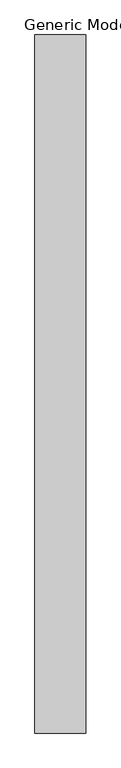
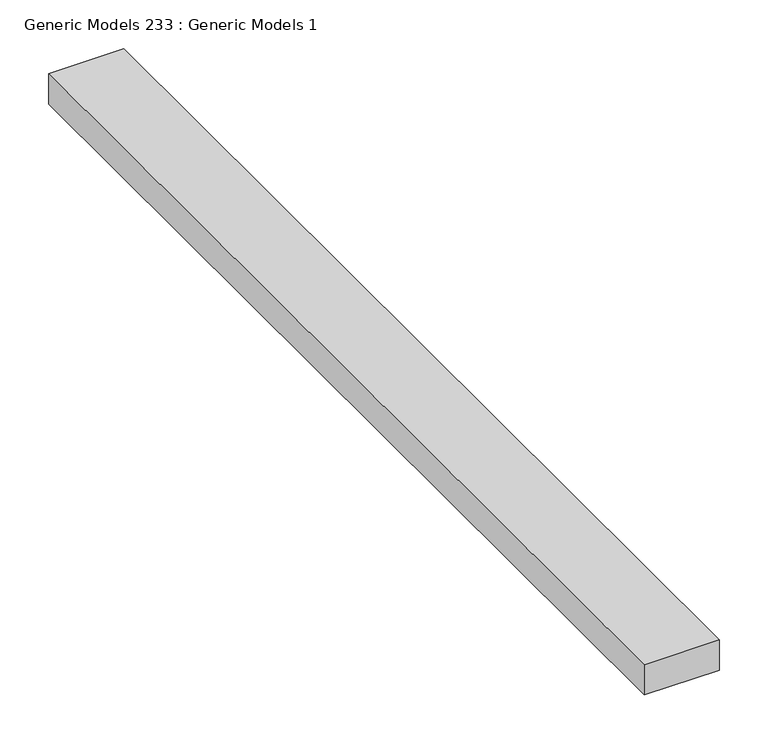
"""IFC4 building model written with IfcOpenShell, lengths in millimetres: proxy geometry, Generic Models 233 : Generic Models 1."""

from ifc_helpers import new_model, si_unit, frame, origin, place, context, project, spatial, polyline, outline, extrude, source, transform, mapped, element, save


def generic_models_233_generic_models_1_ae5bae41(model_context):
    return source(origin(), model_context, "Body", "SweptSolid", [
        extrude(outline(polyline([(48564.8, 0.0), (48475.9, 0.0), (48475.9, 1219.2), (48564.8, 1219.2), (48564.8, 0.0)])), frame((0.0, 0.0, 5467.35), z_axis=(0.0, 0.0, 1.0), x_axis=(1.0, 0.0, 0.0)), (0.0, 0.0, 1.0), 38.1),
    ])


if __name__ == "__main__":
    model = new_model("IFC4")
    model_context = context("Model", 3, world=origin())
    ifc_project = project(units=[si_unit("LENGTHUNIT", "METRE", prefix="MILLI")], contexts=[model_context])
    site = spatial("IfcSite", under=ifc_project)
    building = spatial("IfcBuilding", under=site)
    placement = place(None, origin())
    generic_models_233_generic_models_1_shape = generic_models_233_generic_models_1_ae5bae41(model_context)
    element("IfcBuildingElementProxy", 1, Name="Generic Models 233 : Generic Models 1", ObjectType="Generic Models 233 : Generic Models 1", at=placement, inside=building, context=model_context, shape_type="MappedRepresentation", body=[
        mapped(generic_models_233_generic_models_1_shape, transform((0.0, 0.0, 0.0), x_axis=(1.0, 0.0, 0.0), y_axis=(0.0, 1.0, 0.0), z_axis=(0.0, 0.0, 1.0))),
    ])
    save(model, "model.ifc")

# Revit data of these elements
# Element 1 (IfcBuildingElementProxy, "Generic Models 233 : Generic Models 1")
#   Materials on its faces: "2X WOOD HEADER ATTACHED TO STEEL PURLIN"
# Materials
#   "2X WOOD HEADER ATTACHED TO STEEL PURLIN": class "Wood", colour RGB 234 198 147, transparency 0, Description = "Pinus Echinata", Cost = 0
